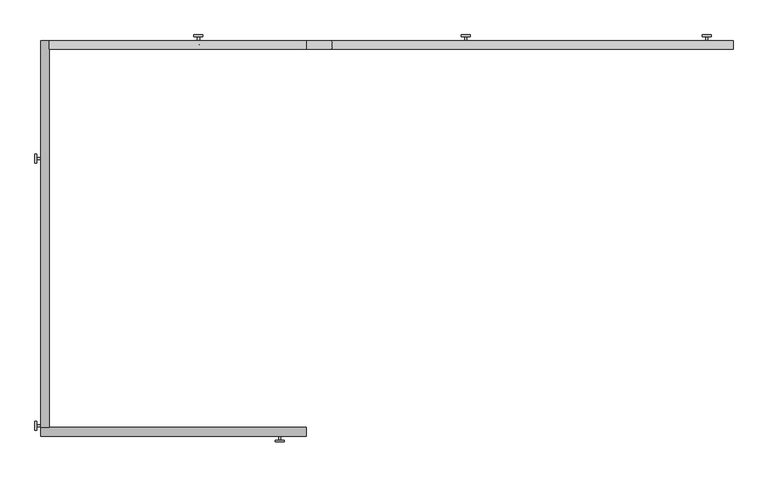
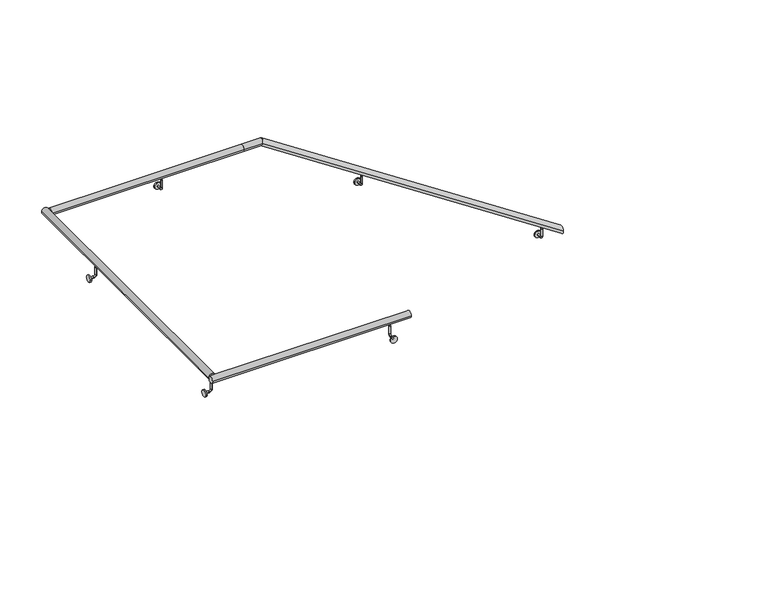
"""IFC4 building model written with IfcOpenShell, lengths in millimetres: railing geometry."""

from ifc_helpers import new_model, si_unit, point, frame, frame_2d, origin, place, context, project, spatial, circle_curve, ellipse_curve, trimmed, segment, composite_curve, outline, extrude, source, transform, mapped, element, save
from ifc_brep_helpers import plane_surface, cylinder_surface, revolved_surface, advanced_brep


def railing_9a7f1ff8(model_context):
    return source(origin(), model_context, "Body", "SolidModel", [
        advanced_brep(
        [(-47571.8499394, -5172.6994487, 1246.5391039), (-47571.8499394, -5122.6994487, 1246.5391039), (-49859.4499252, -5172.6994487, 2752.7777778), (-49859.4499252, -5122.6994487, 2752.7777778), (-50001.8499394, -5172.6994487, 2752.7777778), (-50001.8499394, -5122.6994487, 2752.7777778)],
        [
            (0, 1, ellipse_curve(frame((-47571.8499394, -5147.6994487, 1246.5391039), z_axis=(1.0, 0.0, 0.0), x_axis=(0.0, 0.0, -1.0)), 29.9326144, 25.0)),
            (1, 0, ellipse_curve(frame((-47571.8499394, -5147.6994487, 1246.5391039), z_axis=(1.0, 0.0, 0.0), x_axis=(0.0, 0.0, -1.0)), 29.9326144, 25.0)),
            (0, 2),
            (2, 3, ellipse_curve(frame((-49859.4499252, -5147.6994487, 2752.7777778), z_axis=(0.9579168464509247, 0.0, -0.28704584178405307), x_axis=(-0.2870458417840529, 0.0, -0.9579168464509247)), 26.0982987, 25.0)),
            (3, 1),
            (3, 2, ellipse_curve(frame((-49859.4499252, -5147.6994487, 2752.7777778), z_axis=(0.9579168464509247, 0.0, -0.28704584178405307), x_axis=(-0.2870458417840529, 0.0, -0.9579168464509247)), 26.0982987, 25.0)),
            (4, 5, circle_curve(frame((-50001.8499394, -5147.6994487, 2752.7777778), z_axis=(-1.0, 0.0, 0.0), x_axis=(0.0, 1.0, 0.0)), 25.0)),
            (5, 4, circle_curve(frame((-50001.8499394, -5147.6994487, 2752.7777778), z_axis=(-1.0, 0.0, 0.0), x_axis=(0.0, 1.0, 0.0)), 25.0)),
            (2, 4),
            (5, 3),
        ],
        [
            plane_surface(frame((-47571.8499394, -5147.6994487, 1276.4717183), z_axis=(1.0, 0.0, 0.0), x_axis=(0.0, -1.0, 0.0))),
            cylinder_surface(frame((-47585.5982417, -5147.6994487, 1255.5914841), z_axis=(0.8352093694289688, 0.0, -0.5499320950972624), x_axis=(0.0, 1.0, 0.0)), 25.0),
            plane_surface(frame((-50001.8499394, -5147.6994487, 2777.7777778), z_axis=(-1.0, 0.0, 0.0), x_axis=(0.0, -1.0, 0.0))),
            cylinder_surface(frame((-49851.9585171, -5147.6994487, 2752.7777778), z_axis=(1.0, 0.0, 0.0), x_axis=(0.0, 1.0, 0.0)), 25.0),
        ],
        [
            (0, [[1, 2]]),
            (1, [[-1, 3, 4, 5]]),
            (1, [[-2, -5, 6, -3]]),
            (2, [[7, 8]]),
            (3, [[-4, 9, -8, 10]]),
            (3, [[-6, -10, -7, -9]]),
        ],
    ),
        advanced_brep(
        [(-50001.8499394, -5172.6994487, 2752.7777778), (-50001.8499394, -5122.6994487, 2752.7777778), (-51463.5128792, -5172.6994487, 2752.7777778), (-51463.5128792, -5122.6994487, 2752.7777778)],
        [
            (0, 1, circle_curve(frame((-50001.8499394, -5147.6994487, 2752.7777778), z_axis=(1.0, 0.0, 0.0), x_axis=(0.0, 1.0, 0.0)), 25.0)),
            (1, 0, circle_curve(frame((-50001.8499394, -5147.6994487, 2752.7777778), z_axis=(1.0, 0.0, 0.0), x_axis=(0.0, 1.0, 0.0)), 25.0)),
            (2, 3, circle_curve(frame((-51463.5128792, -5147.6994487, 2752.7777778), z_axis=(-1.0, 0.0, 0.0), x_axis=(0.0, 1.0, 0.0)), 25.0)),
            (3, 2, circle_curve(frame((-51463.5128792, -5147.6994487, 2752.7777778), z_axis=(-1.0, 0.0, 0.0), x_axis=(0.0, 1.0, 0.0)), 25.0)),
            (0, 2),
            (3, 1),
        ],
        [
            plane_surface(frame((-50001.8499394, -5147.6994487, 2777.7777778), z_axis=(1.0, 0.0, 0.0), x_axis=(0.0, -1.0, 0.0))),
            plane_surface(frame((-51463.5128792, -5147.6994487, 2777.7777778), z_axis=(-1.0, 0.0, 0.0), x_axis=(0.0, -1.0, 0.0))),
            cylinder_surface(frame((-50001.8499394, -5147.6994487, 2752.7777778), z_axis=(1.0, 0.0, 0.0), x_axis=(0.0, 1.0, 0.0)), 25.0),
        ],
        [
            (0, [[1, 2]]),
            (1, [[3, 4]]),
            (2, [[-1, 5, -4, 6]]),
            (2, [[-2, -6, -3, -5]]),
        ],
    ),
        advanced_brep(
        [(-51463.5128792, -5122.6994487, 2752.7777778), (-51513.5128792, -5122.6994487, 2752.7777778), (-51463.5128792, -7327.4994487, 2752.7777778), (-51513.5128792, -7327.4994487, 2752.7777778)],
        [
            (0, 1, circle_curve(frame((-51488.5128792, -5122.6994487, 2752.7777778), z_axis=(0.0, 1.0, 0.0), x_axis=(-1.0, 0.0, 0.0)), 25.0)),
            (1, 0, circle_curve(frame((-51488.5128792, -5122.6994487, 2752.7777778), z_axis=(0.0, 1.0, 0.0), x_axis=(-1.0, 0.0, 0.0)), 25.0)),
            (2, 3, circle_curve(frame((-51488.5128792, -7327.4994487, 2752.7777778), z_axis=(0.0, -1.0, 0.0), x_axis=(-1.0, 0.0, 0.0)), 25.0)),
            (3, 2, circle_curve(frame((-51488.5128792, -7327.4994487, 2752.7777778), z_axis=(0.0, -1.0, 0.0), x_axis=(-1.0, 0.0, 0.0)), 25.0)),
            (0, 2),
            (3, 1),
        ],
        [
            plane_surface(frame((-51488.5128792, -5122.6994487, 2777.7777778), z_axis=(0.0, 1.0, 0.0), x_axis=(0.0, 0.0, -1.0))),
            plane_surface(frame((-51488.5128792, -7327.4994487, 2777.7777778), z_axis=(0.0, -1.0, 0.0), x_axis=(0.0, 0.0, -1.0))),
            cylinder_surface(frame((-51488.5128792, -5122.6994487, 2752.7777778), z_axis=(0.0, 1.0, 0.0), x_axis=(-1.0, 0.0, 0.0)), 25.0),
        ],
        [
            (0, [[1, 2]]),
            (1, [[3, 4]]),
            (2, [[-1, 5, -4, 6]]),
            (2, [[-2, -6, -3, -5]]),
        ],
    ),
        advanced_brep(
        [(-51513.5128792, -7327.4994487, 2752.7777778), (-51513.5128792, -7377.4994487, 2752.7777778), (-50001.8499394, -7327.4994487, 2752.7777778), (-50001.8499394, -7377.4994487, 2752.7777778)],
        [
            (0, 1, circle_curve(frame((-51513.5128792, -7352.4994487, 2752.7777778), z_axis=(-1.0, 0.0, 0.0), x_axis=(0.0, -1.0, 0.0)), 25.0)),
            (1, 0, circle_curve(frame((-51513.5128792, -7352.4994487, 2752.7777778), z_axis=(-1.0, 0.0, 0.0), x_axis=(0.0, -1.0, 0.0)), 25.0)),
            (2, 3, circle_curve(frame((-50001.8499394, -7352.4994487, 2752.7777778), z_axis=(1.0, 0.0, 0.0), x_axis=(0.0, -1.0, 0.0)), 25.0)),
            (3, 2, circle_curve(frame((-50001.8499394, -7352.4994487, 2752.7777778), z_axis=(1.0, 0.0, 0.0), x_axis=(0.0, -1.0, 0.0)), 25.0)),
            (0, 2),
            (3, 1),
        ],
        [
            plane_surface(frame((-51513.5128792, -7352.4994487, 2777.7777778), z_axis=(-1.0, 0.0, 0.0), x_axis=(0.0, 1.0, 0.0))),
            plane_surface(frame((-50001.8499394, -7352.4994487, 2777.7777778), z_axis=(1.0, 0.0, 0.0), x_axis=(0.0, 1.0, 0.0))),
            cylinder_surface(frame((-51513.5128792, -7352.4994487, 2752.7777778), z_axis=(-1.0, 0.0, 0.0), x_axis=(0.0, -1.0, 0.0)), 25.0),
        ],
        [
            (0, [[1, 2]]),
            (1, [[3, 4]]),
            (2, [[-1, 5, -4, 6]]),
            (2, [[-2, -6, -3, -5]]),
        ],
    ),
        advanced_brep(
        [(-51488.5128792, -7311.1872126, 2708.7277778), (-51488.5128792, -7323.8872126, 2708.7277778), (-51488.5128792, -7311.1872126, 2651.5777778), (-51488.5128792, -7323.8872126, 2651.5777778), (-51507.5628792, -7323.8872126, 2632.5277778), (-51507.5628792, -7311.1872126, 2632.5277778), (-51536.1378792, -7311.1872126, 2632.5277778), (-51536.1378792, -7323.8872126, 2632.5277778)],
        [
            (0, 1, circle_curve(frame((-51488.5128792, -7317.5372126, 2708.7277778), z_axis=(0.0, 0.0, 1.0), x_axis=(0.0, -1.0, 0.0)), 6.35)),
            (1, 0, circle_curve(frame((-51488.5128792, -7317.5372126, 2708.7277778), z_axis=(0.0, 0.0, 1.0), x_axis=(0.0, -1.0, 0.0)), 6.35)),
            (0, 2),
            (2, 3, circle_curve(frame((-51488.5128792, -7317.5372126, 2651.5777778), z_axis=(0.0, 0.0, 1.0), x_axis=(0.0, -1.0, 0.0)), 6.35)),
            (3, 1),
            (3, 2, circle_curve(frame((-51488.5128792, -7317.5372126, 2651.5777778), z_axis=(0.0, 0.0, 1.0), x_axis=(0.0, -1.0, 0.0)), 6.35)),
            (4, 3, circle_curve(frame((-51507.5628792, -7323.8872126, 2651.5777778), z_axis=(0.0, -1.0, 0.0), x_axis=(1.0, 0.0, 0.0)), 19.05)),
            (2, 5, circle_curve(frame((-51507.5628792, -7311.1872126, 2651.5777778), z_axis=(0.0, 1.0, 0.0), x_axis=(1.0, 0.0, 0.0)), 19.05)),
            (5, 4, circle_curve(frame((-51507.5628792, -7317.5372126, 2632.5277778), z_axis=(1.0, 0.0, 0.0), x_axis=(0.0, -1.0, 0.0)), 6.35)),
            (4, 5, circle_curve(frame((-51507.5628792, -7317.5372126, 2632.5277778), z_axis=(1.0, 0.0, 0.0), x_axis=(0.0, -1.0, 0.0)), 6.35)),
            (6, 7, circle_curve(frame((-51536.1378792, -7317.5372126, 2632.5277778), z_axis=(-1.0, 0.0, 0.0), x_axis=(0.0, -1.0, 0.0)), 6.35)),
            (7, 6, circle_curve(frame((-51536.1378792, -7317.5372126, 2632.5277778), z_axis=(-1.0, 0.0, 0.0), x_axis=(0.0, -1.0, 0.0)), 6.35)),
            (5, 6),
            (7, 4),
        ],
        [
            plane_surface(frame((-51488.5128792, -7323.8872126, 2708.7277778), z_axis=(0.0, 0.0, 1.0), x_axis=(-1.0, 0.0, 0.0))),
            cylinder_surface(frame((-51488.5128792, -7317.5372126, 2708.7277778), z_axis=(0.0, 0.0, 1.0), x_axis=(0.0, -1.0, 0.0)), 6.35),
            revolved_surface(trimmed(ellipse_curve(frame((-51488.5128792, -7317.5372126, 2651.5777778), z_axis=(0.0, 0.0, 1.0), x_axis=(0.0, -1.0, 0.0)), 6.35, 6.35), [point((-51488.5128792, -7311.1872126, 2651.5777778))], [point((-51488.5128792, -7323.8872126, 2651.5777778))], True, "CARTESIAN"), (-51507.5628792, -7317.5372126, 2651.5777778), (0.0, 1.0, 0.0)),
            revolved_surface(trimmed(ellipse_curve(frame((-51488.5128792, -7317.5372126, 2651.5777778), z_axis=(0.0, 0.0, 1.0), x_axis=(0.0, -1.0, 0.0)), 6.35, 6.35), [point((-51488.5128792, -7323.8872126, 2651.5777778))], [point((-51488.5128792, -7311.1872126, 2651.5777778))], True, "CARTESIAN"), (-51507.5628792, -7317.5372126, 2651.5777778), (0.0, 1.0, 0.0)),
            plane_surface(frame((-51536.1378792, -7317.5372126, 2626.1777778), z_axis=(-1.0, 0.0, 0.0), x_axis=(0.0, -1.0, 0.0))),
            cylinder_surface(frame((-51507.5628792, -7317.5372126, 2632.5277778), z_axis=(1.0, 0.0, 0.0), x_axis=(0.0, -1.0, 0.0)), 6.35),
        ],
        [
            (0, [[1, 2]]),
            (1, [[-1, 3, 4, 5]]),
            (1, [[-2, -5, 6, -3]]),
            (2, [[7, -4, 8, 9]]),
            (3, [[-8, -6, -7, 10]]),
            (4, [[11, 12]]),
            (5, [[-9, 13, -12, 14]]),
            (5, [[-10, -14, -11, -13]]),
        ],
    ),
        extrude(outline(composite_curve([segment(trimmed(circle_curve(frame_2d((-7317.5372126, 2632.5277778)), 25.4), [point((-7342.9372126, 2632.5277778))], [point((-7292.1372126, 2632.5277778))], False, "CARTESIAN"), True, "CONTINUOUS"), segment(trimmed(circle_curve(frame_2d((-7317.5372126, 2632.5277778)), 25.4), [point((-7292.1372126, 2632.5277778))], [point((-7342.9372126, 2632.5277778))], False, "CARTESIAN"), True, "CONTINUOUS")], self_intersect=False)), frame((-51545.6628792, 0.0, 0.0), z_axis=(1.0, 0.0, 0.0), x_axis=(0.0, 1.0, 0.0)), (0.0, 0.0, 1.0), 9.525),
        advanced_brep(
        [(-51488.5128792, -5789.5620366, 2708.7277778), (-51488.5128792, -5802.2620366, 2708.7277778), (-51488.5128792, -5789.5620366, 2651.5777778), (-51488.5128792, -5802.2620366, 2651.5777778), (-51507.5628792, -5802.2620366, 2632.5277778), (-51507.5628792, -5789.5620366, 2632.5277778), (-51536.1378792, -5789.5620366, 2632.5277778), (-51536.1378792, -5802.2620366, 2632.5277778)],
        [
            (0, 1, circle_curve(frame((-51488.5128792, -5795.9120366, 2708.7277778), z_axis=(0.0, 0.0, 1.0), x_axis=(0.0, -1.0, 0.0)), 6.35)),
            (1, 0, circle_curve(frame((-51488.5128792, -5795.9120366, 2708.7277778), z_axis=(0.0, 0.0, 1.0), x_axis=(0.0, -1.0, 0.0)), 6.35)),
            (0, 2),
            (2, 3, circle_curve(frame((-51488.5128792, -5795.9120366, 2651.5777778), z_axis=(0.0, 0.0, 1.0), x_axis=(0.0, -1.0, 0.0)), 6.35)),
            (3, 1),
            (3, 2, circle_curve(frame((-51488.5128792, -5795.9120366, 2651.5777778), z_axis=(0.0, 0.0, 1.0), x_axis=(0.0, -1.0, 0.0)), 6.35)),
            (4, 3, circle_curve(frame((-51507.5628792, -5802.2620366, 2651.5777778), z_axis=(0.0, -1.0, 0.0), x_axis=(1.0, 0.0, 0.0)), 19.05)),
            (2, 5, circle_curve(frame((-51507.5628792, -5789.5620366, 2651.5777778), z_axis=(0.0, 1.0, 0.0), x_axis=(1.0, 0.0, 0.0)), 19.05)),
            (5, 4, circle_curve(frame((-51507.5628792, -5795.9120366, 2632.5277778), z_axis=(1.0, 0.0, 0.0), x_axis=(0.0, -1.0, 0.0)), 6.35)),
            (4, 5, circle_curve(frame((-51507.5628792, -5795.9120366, 2632.5277778), z_axis=(1.0, 0.0, 0.0), x_axis=(0.0, -1.0, 0.0)), 6.35)),
            (6, 7, circle_curve(frame((-51536.1378792, -5795.9120366, 2632.5277778), z_axis=(-1.0, 0.0, 0.0), x_axis=(0.0, -1.0, 0.0)), 6.35)),
            (7, 6, circle_curve(frame((-51536.1378792, -5795.9120366, 2632.5277778), z_axis=(-1.0, 0.0, 0.0), x_axis=(0.0, -1.0, 0.0)), 6.35)),
            (5, 6),
            (7, 4),
        ],
        [
            plane_surface(frame((-51488.5128792, -5802.2620366, 2708.7277778), z_axis=(0.0, 0.0, 1.0), x_axis=(-1.0, 0.0, 0.0))),
            cylinder_surface(frame((-51488.5128792, -5795.9120366, 2708.7277778), z_axis=(0.0, 0.0, 1.0), x_axis=(0.0, -1.0, 0.0)), 6.35),
            revolved_surface(trimmed(ellipse_curve(frame((-51488.5128792, -5795.9120366, 2651.5777778), z_axis=(0.0, 0.0, 1.0), x_axis=(0.0, -1.0, 0.0)), 6.35, 6.35), [point((-51488.5128792, -5789.5620366, 2651.5777778))], [point((-51488.5128792, -5802.2620366, 2651.5777778))], True, "CARTESIAN"), (-51507.5628792, -5795.9120366, 2651.5777778), (0.0, 1.0, 0.0)),
            revolved_surface(trimmed(ellipse_curve(frame((-51488.5128792, -5795.9120366, 2651.5777778), z_axis=(0.0, 0.0, 1.0), x_axis=(0.0, -1.0, 0.0)), 6.35, 6.35), [point((-51488.5128792, -5802.2620366, 2651.5777778))], [point((-51488.5128792, -5789.5620366, 2651.5777778))], True, "CARTESIAN"), (-51507.5628792, -5795.9120366, 2651.5777778), (0.0, 1.0, 0.0)),
            plane_surface(frame((-51536.1378792, -5795.9120366, 2626.1777778), z_axis=(-1.0, 0.0, 0.0), x_axis=(0.0, -1.0, 0.0))),
            cylinder_surface(frame((-51507.5628792, -5795.9120366, 2632.5277778), z_axis=(1.0, 0.0, 0.0), x_axis=(0.0, -1.0, 0.0)), 6.35),
        ],
        [
            (0, [[1, 2]]),
            (1, [[-1, 3, 4, 5]]),
            (1, [[-2, -5, 6, -3]]),
            (2, [[7, -4, 8, 9]]),
            (3, [[-8, -6, -7, 10]]),
            (4, [[11, 12]]),
            (5, [[-9, 13, -12, 14]]),
            (5, [[-10, -14, -11, -13]]),
        ],
    ),
        extrude(outline(composite_curve([segment(trimmed(circle_curve(frame_2d((-5795.9120366, 2632.5277778)), 25.4), [point((-5821.3120366, 2632.5277778))], [point((-5770.5120366, 2632.5277778))], False, "CARTESIAN"), True, "CONTINUOUS"), segment(trimmed(circle_curve(frame_2d((-5795.9120366, 2632.5277778)), 25.4), [point((-5770.5120366, 2632.5277778))], [point((-5821.3120366, 2632.5277778))], False, "CARTESIAN"), True, "CONTINUOUS")], self_intersect=False)), frame((-51545.6628792, 0.0, 0.0), z_axis=(1.0, 0.0, 0.0), x_axis=(0.0, 1.0, 0.0)), (0.0, 0.0, 1.0), 9.525),
        advanced_brep(
        [(-50608.7502912, -5147.6994487, 2708.7277778), (-50621.4502912, -5147.6994487, 2708.7277778), (-50608.7502912, -5147.6994487, 2651.5777778), (-50621.4502912, -5147.6994487, 2651.5777778), (-50621.4502912, -5128.6494487, 2632.5277778), (-50608.7502912, -5128.6494487, 2632.5277778), (-50608.7502912, -5100.0744487, 2632.5277778), (-50621.4502912, -5100.0744487, 2632.5277778)],
        [
            (0, 1, circle_curve(frame((-50615.1002912, -5147.6994487, 2708.7277778), z_axis=(0.0, 0.0, 1.0), x_axis=(-1.0, 0.0, 0.0)), 6.35)),
            (1, 0, circle_curve(frame((-50615.1002912, -5147.6994487, 2708.7277778), z_axis=(0.0, 0.0, 1.0), x_axis=(-1.0, 0.0, 0.0)), 6.35)),
            (0, 2),
            (2, 3, circle_curve(frame((-50615.1002912, -5147.6994487, 2651.5777778), z_axis=(0.0, 0.0, 1.0), x_axis=(-1.0, 0.0, 0.0)), 6.35)),
            (3, 1),
            (3, 2, circle_curve(frame((-50615.1002912, -5147.6994487, 2651.5777778), z_axis=(0.0, 0.0, 1.0), x_axis=(-1.0, 0.0, 0.0)), 6.35)),
            (4, 3, circle_curve(frame((-50621.4502912, -5128.6494487, 2651.5777778), z_axis=(-1.0, 0.0, 0.0), x_axis=(0.0, -1.0, 0.0)), 19.05)),
            (2, 5, circle_curve(frame((-50608.7502912, -5128.6494487, 2651.5777778), z_axis=(1.0, 0.0, 0.0), x_axis=(0.0, -1.0, 0.0)), 19.05)),
            (5, 4, circle_curve(frame((-50615.1002912, -5128.6494487, 2632.5277778), z_axis=(0.0, -1.0, 0.0), x_axis=(-1.0, 0.0, 0.0)), 6.35)),
            (4, 5, circle_curve(frame((-50615.1002912, -5128.6494487, 2632.5277778), z_axis=(0.0, -1.0, 0.0), x_axis=(-1.0, 0.0, 0.0)), 6.35)),
            (6, 7, circle_curve(frame((-50615.1002912, -5100.0744487, 2632.5277778), z_axis=(0.0, 1.0, 0.0), x_axis=(-1.0, 0.0, 0.0)), 6.35)),
            (7, 6, circle_curve(frame((-50615.1002912, -5100.0744487, 2632.5277778), z_axis=(0.0, 1.0, 0.0), x_axis=(-1.0, 0.0, 0.0)), 6.35)),
            (5, 6),
            (7, 4),
        ],
        [
            plane_surface(frame((-50621.4502912, -5147.6994487, 2708.7277778), z_axis=(0.0, 0.0, 1.0), x_axis=(0.0, 1.0, 0.0))),
            cylinder_surface(frame((-50615.1002912, -5147.6994487, 2708.7277778), z_axis=(0.0, 0.0, 1.0), x_axis=(-1.0, 0.0, 0.0)), 6.35),
            revolved_surface(trimmed(ellipse_curve(frame((-50615.1002912, -5147.6994487, 2651.5777778), z_axis=(0.0, 0.0, 1.0), x_axis=(-1.0, 0.0, 0.0)), 6.35, 6.35), [point((-50608.7502912, -5147.6994487, 2651.5777778))], [point((-50621.4502912, -5147.6994487, 2651.5777778))], True, "CARTESIAN"), (-50615.1002912, -5128.6494487, 2651.5777778), (1.0, 0.0, 0.0)),
            revolved_surface(trimmed(ellipse_curve(frame((-50615.1002912, -5147.6994487, 2651.5777778), z_axis=(0.0, 0.0, 1.0), x_axis=(-1.0, 0.0, 0.0)), 6.35, 6.35), [point((-50621.4502912, -5147.6994487, 2651.5777778))], [point((-50608.7502912, -5147.6994487, 2651.5777778))], True, "CARTESIAN"), (-50615.1002912, -5128.6494487, 2651.5777778), (1.0, 0.0, 0.0)),
            plane_surface(frame((-50615.1002912, -5100.0744487, 2626.1777778), z_axis=(0.0, 1.0, 0.0), x_axis=(-1.0, 0.0, 0.0))),
            cylinder_surface(frame((-50615.1002912, -5128.6494487, 2632.5277778), z_axis=(0.0, -1.0, 0.0), x_axis=(-1.0, 0.0, 0.0)), 6.35),
        ],
        [
            (0, [[1, 2]]),
            (1, [[-1, 3, 4, 5]]),
            (1, [[-2, -5, 6, -3]]),
            (2, [[7, -4, 8, 9]]),
            (3, [[-8, -6, -7, 10]]),
            (4, [[11, 12]]),
            (5, [[-9, 13, -12, 14]]),
            (5, [[-10, -14, -11, -13]]),
        ],
    ),
        extrude(outline(composite_curve([segment(trimmed(circle_curve(frame_2d((2632.5277778, -50615.1002912)), 25.4), [point((2632.5277778, -50640.5002912))], [point((2632.5277778, -50589.7002912))], False, "CARTESIAN"), True, "CONTINUOUS"), segment(trimmed(circle_curve(frame_2d((2632.5277778, -50615.1002912)), 25.4), [point((2632.5277778, -50589.7002912))], [point((2632.5277778, -50640.5002912))], False, "CARTESIAN"), True, "CONTINUOUS")], self_intersect=False)), frame((0.0, -5100.0744487, 0.0), z_axis=(0.0, 1.0, 0.0), x_axis=(0.0, 0.0, 1.0)), (0.0, 0.0, 1.0), 9.525),
        advanced_brep(
        [(-49087.1251153, -5147.6994487, 2209.3148383), (-49099.8251153, -5147.6994487, 2209.3148383), (-49087.1251153, -5147.6994487, 2152.1648383), (-49099.8251153, -5147.6994487, 2152.1648383), (-49099.8251153, -5128.6494487, 2133.1148383), (-49087.1251153, -5128.6494487, 2133.1148383), (-49087.1251153, -5100.0744487, 2133.1148383), (-49099.8251153, -5100.0744487, 2133.1148383)],
        [
            (0, 1, circle_curve(frame((-49093.4751153, -5147.6994487, 2209.3148383), z_axis=(0.0, 0.0, 1.0), x_axis=(-1.0, 0.0, 0.0)), 6.35)),
            (1, 0, circle_curve(frame((-49093.4751153, -5147.6994487, 2209.3148383), z_axis=(0.0, 0.0, 1.0), x_axis=(-1.0, 0.0, 0.0)), 6.35)),
            (0, 2),
            (2, 3, circle_curve(frame((-49093.4751153, -5147.6994487, 2152.1648383), z_axis=(0.0, 0.0, 1.0), x_axis=(-1.0, 0.0, 0.0)), 6.35)),
            (3, 1),
            (3, 2, circle_curve(frame((-49093.4751153, -5147.6994487, 2152.1648383), z_axis=(0.0, 0.0, 1.0), x_axis=(-1.0, 0.0, 0.0)), 6.35)),
            (4, 3, circle_curve(frame((-49099.8251153, -5128.6494487, 2152.1648383), z_axis=(-1.0, 0.0, 0.0), x_axis=(0.0, -1.0, 0.0)), 19.05)),
            (2, 5, circle_curve(frame((-49087.1251153, -5128.6494487, 2152.1648383), z_axis=(1.0, 0.0, 0.0), x_axis=(0.0, -1.0, 0.0)), 19.05)),
            (5, 4, circle_curve(frame((-49093.4751153, -5128.6494487, 2133.1148383), z_axis=(0.0, -1.0, 0.0), x_axis=(-1.0, 0.0, 0.0)), 6.35)),
            (4, 5, circle_curve(frame((-49093.4751153, -5128.6494487, 2133.1148383), z_axis=(0.0, -1.0, 0.0), x_axis=(-1.0, 0.0, 0.0)), 6.35)),
            (6, 7, circle_curve(frame((-49093.4751153, -5100.0744487, 2133.1148383), z_axis=(0.0, 1.0, 0.0), x_axis=(-1.0, 0.0, 0.0)), 6.35)),
            (7, 6, circle_curve(frame((-49093.4751153, -5100.0744487, 2133.1148383), z_axis=(0.0, 1.0, 0.0), x_axis=(-1.0, 0.0, 0.0)), 6.35)),
            (5, 6),
            (7, 4),
        ],
        [
            plane_surface(frame((-49099.8251153, -5147.6994487, 2209.3148383), z_axis=(0.0, 0.0, 1.0), x_axis=(0.0, 1.0, 0.0))),
            cylinder_surface(frame((-49093.4751153, -5147.6994487, 2209.3148383), z_axis=(0.0, 0.0, 1.0), x_axis=(-1.0, 0.0, 0.0)), 6.35),
            revolved_surface(trimmed(ellipse_curve(frame((-49093.4751153, -5147.6994487, 2152.1648383), z_axis=(0.0, 0.0, 1.0), x_axis=(-1.0, 0.0, 0.0)), 6.35, 6.35), [point((-49087.1251153, -5147.6994487, 2152.1648383))], [point((-49099.8251153, -5147.6994487, 2152.1648383))], True, "CARTESIAN"), (-49093.4751153, -5128.6494487, 2152.1648383), (1.0, 0.0, 0.0)),
            revolved_surface(trimmed(ellipse_curve(frame((-49093.4751153, -5147.6994487, 2152.1648383), z_axis=(0.0, 0.0, 1.0), x_axis=(-1.0, 0.0, 0.0)), 6.35, 6.35), [point((-49099.8251153, -5147.6994487, 2152.1648383))], [point((-49087.1251153, -5147.6994487, 2152.1648383))], True, "CARTESIAN"), (-49093.4751153, -5128.6494487, 2152.1648383), (1.0, 0.0, 0.0)),
            plane_surface(frame((-49093.4751153, -5100.0744487, 2126.7648383), z_axis=(0.0, 1.0, 0.0), x_axis=(-1.0, 0.0, 0.0))),
            cylinder_surface(frame((-49093.4751153, -5128.6494487, 2133.1148383), z_axis=(0.0, -1.0, 0.0), x_axis=(-1.0, 0.0, 0.0)), 6.35),
        ],
        [
            (0, [[1, 2]]),
            (1, [[-1, 3, 4, 5]]),
            (1, [[-2, -5, 6, -3]]),
            (2, [[7, -4, 8, 9]]),
            (3, [[-8, -6, -7, 10]]),
            (4, [[11, 12]]),
            (5, [[-9, 13, -12, 14]]),
            (5, [[-10, -14, -11, -13]]),
        ],
    ),
        extrude(outline(composite_curve([segment(trimmed(circle_curve(frame_2d((2133.1148383, -49093.4751153)), 25.4), [point((2133.1148383, -49118.8751153))], [point((2133.1148383, -49068.0751153))], False, "CARTESIAN"), True, "CONTINUOUS"), segment(trimmed(circle_curve(frame_2d((2133.1148383, -49093.4751153)), 25.4), [point((2133.1148383, -49068.0751153))], [point((2133.1148383, -49118.8751153))], False, "CARTESIAN"), True, "CONTINUOUS")], self_intersect=False)), frame((0.0, -5100.0744487, 0.0), z_axis=(0.0, 1.0, 0.0), x_axis=(0.0, 0.0, 1.0)), (0.0, 0.0, 1.0), 9.525),
        advanced_brep(
        [(-50158.1999394, -7352.4994487, 2708.7277778), (-50145.4999394, -7352.4994487, 2708.7277778), (-50158.1999394, -7352.4994487, 2651.5777778), (-50145.4999394, -7352.4994487, 2651.5777778), (-50145.4999394, -7371.5494487, 2632.5277778), (-50158.1999394, -7371.5494487, 2632.5277778), (-50158.1999394, -7400.1244487, 2632.5277778), (-50145.4999394, -7400.1244487, 2632.5277778)],
        [
            (0, 1, circle_curve(frame((-50151.8499394, -7352.4994487, 2708.7277778), z_axis=(0.0, 0.0, 1.0), x_axis=(1.0, 0.0, 0.0)), 6.35)),
            (1, 0, circle_curve(frame((-50151.8499394, -7352.4994487, 2708.7277778), z_axis=(0.0, 0.0, 1.0), x_axis=(1.0, 0.0, 0.0)), 6.35)),
            (0, 2),
            (2, 3, circle_curve(frame((-50151.8499394, -7352.4994487, 2651.5777778), z_axis=(0.0, 0.0, 1.0), x_axis=(1.0, 0.0, 0.0)), 6.35)),
            (3, 1),
            (3, 2, circle_curve(frame((-50151.8499394, -7352.4994487, 2651.5777778), z_axis=(0.0, 0.0, 1.0), x_axis=(1.0, 0.0, 0.0)), 6.35)),
            (4, 3, circle_curve(frame((-50145.4999394, -7371.5494487, 2651.5777778), z_axis=(1.0, 0.0, 0.0), x_axis=(0.0, 1.0, 0.0)), 19.05)),
            (2, 5, circle_curve(frame((-50158.1999394, -7371.5494487, 2651.5777778), z_axis=(-1.0, 0.0, 0.0), x_axis=(0.0, 1.0, 0.0)), 19.05)),
            (5, 4, circle_curve(frame((-50151.8499394, -7371.5494487, 2632.5277778), z_axis=(0.0, 1.0, 0.0), x_axis=(1.0, 0.0, 0.0)), 6.35)),
            (4, 5, circle_curve(frame((-50151.8499394, -7371.5494487, 2632.5277778), z_axis=(0.0, 1.0, 0.0), x_axis=(1.0, 0.0, 0.0)), 6.35)),
            (6, 7, circle_curve(frame((-50151.8499394, -7400.1244487, 2632.5277778), z_axis=(0.0, -1.0, 0.0), x_axis=(1.0, 0.0, 0.0)), 6.35)),
            (7, 6, circle_curve(frame((-50151.8499394, -7400.1244487, 2632.5277778), z_axis=(0.0, -1.0, 0.0), x_axis=(1.0, 0.0, 0.0)), 6.35)),
            (5, 6),
            (7, 4),
        ],
        [
            plane_surface(frame((-50145.4999394, -7352.4994487, 2708.7277778), z_axis=(0.0, 0.0, 1.0), x_axis=(0.0, -1.0, 0.0))),
            cylinder_surface(frame((-50151.8499394, -7352.4994487, 2708.7277778), z_axis=(0.0, 0.0, 1.0), x_axis=(1.0, 0.0, 0.0)), 6.35),
            revolved_surface(trimmed(ellipse_curve(frame((-50151.8499394, -7352.4994487, 2651.5777778), z_axis=(0.0, 0.0, 1.0), x_axis=(1.0, 0.0, 0.0)), 6.35, 6.35), [point((-50158.1999394, -7352.4994487, 2651.5777778))], [point((-50145.4999394, -7352.4994487, 2651.5777778))], True, "CARTESIAN"), (-50151.8499394, -7371.5494487, 2651.5777778), (-1.0, 0.0, 0.0)),
            revolved_surface(trimmed(ellipse_curve(frame((-50151.8499394, -7352.4994487, 2651.5777778), z_axis=(0.0, 0.0, 1.0), x_axis=(1.0, 0.0, 0.0)), 6.35, 6.35), [point((-50145.4999394, -7352.4994487, 2651.5777778))], [point((-50158.1999394, -7352.4994487, 2651.5777778))], True, "CARTESIAN"), (-50151.8499394, -7371.5494487, 2651.5777778), (-1.0, 0.0, 0.0)),
            plane_surface(frame((-50151.8499394, -7400.1244487, 2626.1777778), z_axis=(0.0, -1.0, 0.0), x_axis=(1.0, 0.0, 0.0))),
            cylinder_surface(frame((-50151.8499394, -7371.5494487, 2632.5277778), z_axis=(0.0, 1.0, 0.0), x_axis=(1.0, 0.0, 0.0)), 6.35),
        ],
        [
            (0, [[1, 2]]),
            (1, [[-1, 3, 4, 5]]),
            (1, [[-2, -5, 6, -3]]),
            (2, [[7, -4, 8, 9]]),
            (3, [[-8, -6, -7, 10]]),
            (4, [[11, 12]]),
            (5, [[-9, 13, -12, 14]]),
            (5, [[-10, -14, -11, -13]]),
        ],
    ),
        extrude(outline(composite_curve([segment(trimmed(circle_curve(frame_2d((2632.5277778, -50151.8499394)), 25.4), [point((2632.5277778, -50126.4499394))], [point((2632.5277778, -50177.2499394))], False, "CARTESIAN"), True, "CONTINUOUS"), segment(trimmed(circle_curve(frame_2d((2632.5277778, -50151.8499394)), 25.4), [point((2632.5277778, -50177.2499394))], [point((2632.5277778, -50126.4499394))], False, "CARTESIAN"), True, "CONTINUOUS")], self_intersect=False)), frame((0.0, -7409.6494487, 0.0), z_axis=(0.0, 1.0, 0.0), x_axis=(0.0, 0.0, 1.0)), (0.0, 0.0, 1.0), 9.525),
        advanced_brep(
        [(-47715.4999394, -5147.6994487, 1306.1871504), (-47728.1999394, -5147.6994487, 1306.1871504), (-47715.4999394, -5147.6994487, 1249.0371504), (-47728.1999394, -5147.6994487, 1249.0371504), (-47728.1999394, -5128.6494487, 1229.9871504), (-47715.4999394, -5128.6494487, 1229.9871504), (-47715.4999394, -5100.0744487, 1229.9871504), (-47728.1999394, -5100.0744487, 1229.9871504)],
        [
            (0, 1, circle_curve(frame((-47721.8499394, -5147.6994487, 1306.1871504), z_axis=(0.0, 0.0, 1.0), x_axis=(-1.0, 0.0, 0.0)), 6.35)),
            (1, 0, circle_curve(frame((-47721.8499394, -5147.6994487, 1306.1871504), z_axis=(0.0, 0.0, 1.0), x_axis=(-1.0, 0.0, 0.0)), 6.35)),
            (0, 2),
            (2, 3, circle_curve(frame((-47721.8499394, -5147.6994487, 1249.0371504), z_axis=(0.0, 0.0, 1.0), x_axis=(-1.0, 0.0, 0.0)), 6.35)),
            (3, 1),
            (3, 2, circle_curve(frame((-47721.8499394, -5147.6994487, 1249.0371504), z_axis=(0.0, 0.0, 1.0), x_axis=(-1.0, 0.0, 0.0)), 6.35)),
            (4, 3, circle_curve(frame((-47728.1999394, -5128.6494487, 1249.0371504), z_axis=(-1.0, 0.0, 0.0), x_axis=(0.0, -1.0, 0.0)), 19.05)),
            (2, 5, circle_curve(frame((-47715.4999394, -5128.6494487, 1249.0371504), z_axis=(1.0, 0.0, 0.0), x_axis=(0.0, -1.0, 0.0)), 19.05)),
            (5, 4, circle_curve(frame((-47721.8499394, -5128.6494487, 1229.9871504), z_axis=(0.0, -1.0, 0.0), x_axis=(-1.0, 0.0, 0.0)), 6.35)),
            (4, 5, circle_curve(frame((-47721.8499394, -5128.6494487, 1229.9871504), z_axis=(0.0, -1.0, 0.0), x_axis=(-1.0, 0.0, 0.0)), 6.35)),
            (6, 7, circle_curve(frame((-47721.8499394, -5100.0744487, 1229.9871504), z_axis=(0.0, 1.0, 0.0), x_axis=(-1.0, 0.0, 0.0)), 6.35)),
            (7, 6, circle_curve(frame((-47721.8499394, -5100.0744487, 1229.9871504), z_axis=(0.0, 1.0, 0.0), x_axis=(-1.0, 0.0, 0.0)), 6.35)),
            (5, 6),
            (7, 4),
        ],
        [
            plane_surface(frame((-47728.1999394, -5147.6994487, 1306.1871504), z_axis=(0.0, 0.0, 1.0), x_axis=(0.0, 1.0, 0.0))),
            cylinder_surface(frame((-47721.8499394, -5147.6994487, 1306.1871504), z_axis=(0.0, 0.0, 1.0), x_axis=(-1.0, 0.0, 0.0)), 6.35),
            revolved_surface(trimmed(ellipse_curve(frame((-47721.8499394, -5147.6994487, 1249.0371504), z_axis=(0.0, 0.0, 1.0), x_axis=(-1.0, 0.0, 0.0)), 6.35, 6.35), [point((-47715.4999394, -5147.6994487, 1249.0371504))], [point((-47728.1999394, -5147.6994487, 1249.0371504))], True, "CARTESIAN"), (-47721.8499394, -5128.6494487, 1249.0371504), (1.0, 0.0, 0.0)),
            revolved_surface(trimmed(ellipse_curve(frame((-47721.8499394, -5147.6994487, 1249.0371504), z_axis=(0.0, 0.0, 1.0), x_axis=(-1.0, 0.0, 0.0)), 6.35, 6.35), [point((-47728.1999394, -5147.6994487, 1249.0371504))], [point((-47715.4999394, -5147.6994487, 1249.0371504))], True, "CARTESIAN"), (-47721.8499394, -5128.6494487, 1249.0371504), (1.0, 0.0, 0.0)),
            plane_surface(frame((-47721.8499394, -5100.0744487, 1223.6371504), z_axis=(0.0, 1.0, 0.0), x_axis=(-1.0, 0.0, 0.0))),
            cylinder_surface(frame((-47721.8499394, -5128.6494487, 1229.9871504), z_axis=(0.0, -1.0, 0.0), x_axis=(-1.0, 0.0, 0.0)), 6.35),
        ],
        [
            (0, [[1, 2]]),
            (1, [[-1, 3, 4, 5]]),
            (1, [[-2, -5, 6, -3]]),
            (2, [[7, -4, 8, 9]]),
            (3, [[-8, -6, -7, 10]]),
            (4, [[11, 12]]),
            (5, [[-9, 13, -12, 14]]),
            (5, [[-10, -14, -11, -13]]),
        ],
    ),
        extrude(outline(composite_curve([segment(trimmed(circle_curve(frame_2d((1229.9871504, -47721.8499394)), 25.4), [point((1229.9871504, -47747.2499394))], [point((1229.9871504, -47696.4499394))], False, "CARTESIAN"), True, "CONTINUOUS"), segment(trimmed(circle_curve(frame_2d((1229.9871504, -47721.8499394)), 25.4), [point((1229.9871504, -47696.4499394))], [point((1229.9871504, -47747.2499394))], False, "CARTESIAN"), True, "CONTINUOUS")], self_intersect=False)), frame((0.0, -5100.0744487, 0.0), z_axis=(0.0, 1.0, 0.0), x_axis=(0.0, 0.0, 1.0)), (0.0, 0.0, 1.0), 9.525),
    ])


if __name__ == "__main__":
    model = new_model("IFC4")
    model_context = context("Model", 3, world=origin())
    ifc_project = project(units=[si_unit("LENGTHUNIT", "METRE", prefix="MILLI")], contexts=[model_context])
    site = spatial("IfcSite", under=ifc_project)
    building = spatial("IfcBuilding", under=site)
    placement = place(None, origin())
    railing_shape = railing_9a7f1ff8(model_context)
    element("IfcRailing", 1, at=placement, inside=building, context=model_context, shape_type="MappedRepresentation", body=[
        mapped(railing_shape, transform((0.0, 0.0, 0.0), x_axis=(1.0, 0.0, 0.0), y_axis=(0.0, 1.0, 0.0), z_axis=(0.0, 0.0, 1.0))),
    ])
    save(model, "model.ifc")
